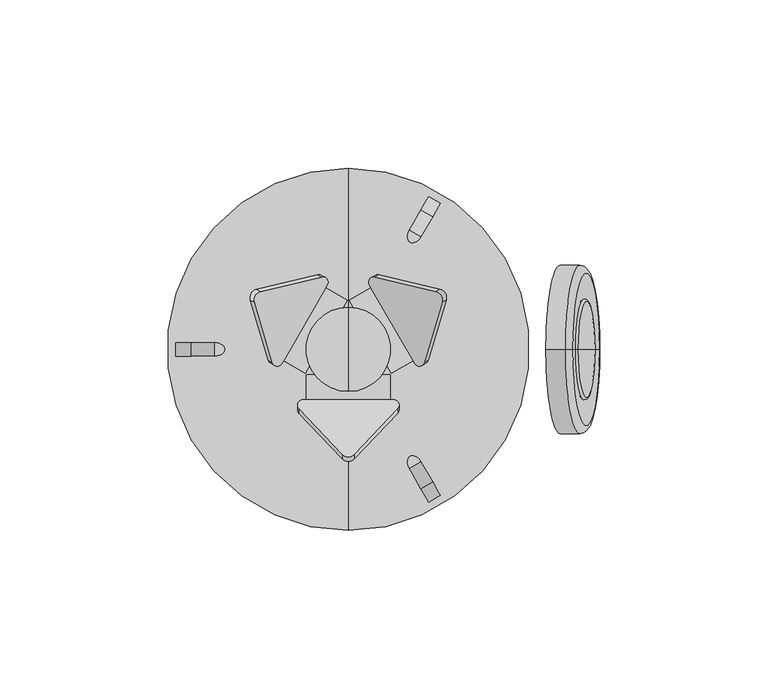
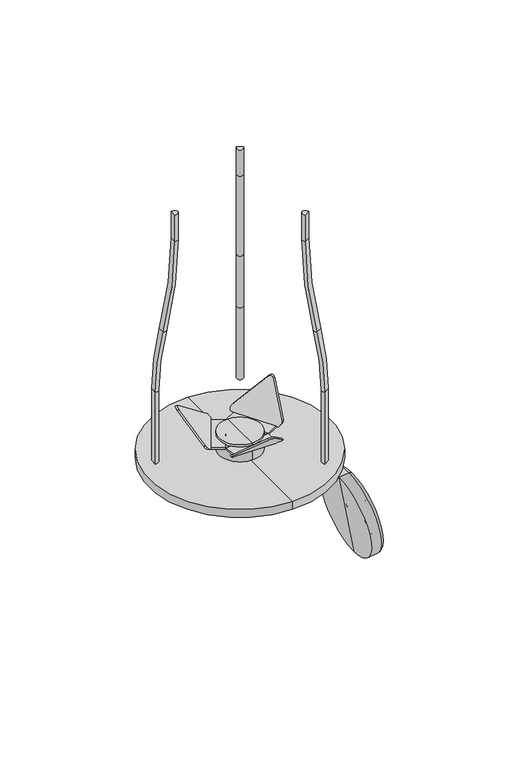
"""IFC4 building model written with IfcOpenShell, lengths in millimetres: proxy geometry, Smoothie_Maker_ : Smoothie_Maker_."""

from ifc_helpers import new_model, si_unit, point, frame, origin, place, context, project, spatial, polyline, circle_curve, ellipse_curve, trimmed, source, transform, mapped, element, save
from ifc_brep_helpers import plane_surface, cylinder_surface, revolved_surface, extruded_surface, advanced_brep


def generic_models_17cbc278(model_context):
    return source(origin(), model_context, "Body", "AdvancedBrep", [
        advanced_brep(
        [(21.5767384, -33.401336, 302.0), (18.1380363, -35.3866715, 302.0), (21.5767384, -33.401336, 285.575084), (18.1380363, -35.3866715, 285.575084), (21.6115055, -41.4028966, 231.2107577), (25.0502075, -39.417561, 231.2107577), (23.9250989, -45.410158, 195.0), (27.363801, -43.4248225, 195.0), (27.363801, -43.4248225, 150.0), (23.9250989, -45.410158, 150.0)],
        [
            (0, 1, ellipse_curve(frame((19.8573873, -34.3940038, 302.0), z_axis=(0.0, 0.0, 1.0), x_axis=(0.5000000000000502, -0.8660254037844097, 0.0)), 2.9839648, 1.9853355)),
            (1, 0),
            (0, 2),
            (2, 3, ellipse_curve(frame((19.8573873, -34.3940038, 285.575084), z_axis=(0.0, 0.0, 1.0), x_axis=(0.5000000000000502, -0.8660254037844097, 0.0)), 2.9839648, 1.9853355)),
            (3, 1),
            (3, 2),
            (4, 3, circle_curve(frame((126.233855, -222.6141215, 285.575084), z_axis=(0.8660254037844424, 0.49999999999999367, 0.0), x_axis=(-0.49999999999999367, 0.8660254037844424, 0.0)), 216.1916373)),
            (2, 5, circle_curve(frame((129.672557, -220.628786, 285.575084), z_axis=(-0.8660254037844424, -0.49999999999999367, 0.0), x_axis=(-0.49999999999999367, 0.8660254037844424, 0.0)), 216.1916373)),
            (5, 4, ellipse_curve(frame((23.3308565, -40.4102288, 231.2107577), z_axis=(-0.1257317975289871, 0.2177738614471723, 0.9678667575449205), x_axis=(0.4839333787725105, -0.838197199512346, 0.25146359505797733)), 2.9839648, 1.9853355)),
            (4, 5),
            (6, 4, circle_curve(frame((-48.0749011, 79.2975001, 195.0), z_axis=(-0.8660254037844424, -0.49999999999999367, 0.0), x_axis=(0.4839333787724538, -0.8381971995123781, 0.25146359505797933)), 144.0)),
            (5, 7, circle_curve(frame((-44.636199, 81.2828357, 195.0), z_axis=(0.8660254037844424, 0.49999999999999367, 0.0), x_axis=(0.4839333787724538, -0.8381971995123781, 0.25146359505797933)), 144.0)),
            (7, 6, ellipse_curve(frame((25.6444499, -44.4174902, 195.0), z_axis=(0.0, 0.0, 1.0), x_axis=(0.5000000000000503, -0.8660254037844097, 0.0)), 2.9839648, 1.9853355)),
            (6, 7),
            (8, 9),
            (9, 8, ellipse_curve(frame((25.6444499, -44.4174902, 150.0), z_axis=(0.0, 0.0, -1.0), x_axis=(0.5000000000000503, -0.8660254037844097, 0.0)), 2.9839648, 1.9853355)),
            (7, 8),
            (9, 6),
        ],
        [
            plane_surface(frame((19.8573873, -34.3940038, 302.0), z_axis=(0.0, 0.0, 1.0), x_axis=(0.8660254037844424, 0.4999999999999936, 0.0))),
            extruded_surface(trimmed(ellipse_curve(frame((19.8573873, -34.3940038, 285.575084), z_axis=(0.0, 0.0, 1.0), x_axis=(0.5000000000000502, -0.8660254037844097, 0.0)), 2.9839648, 1.9853355), [point((21.5767384, -33.401336, 285.575084))], [point((18.1380363, -35.3866715, 285.575084))], True, "CARTESIAN"), (0.0, 0.0, 16.424915999999996), 16.424915999999996),
            plane_surface(frame((18.1380363, -35.3866715, 302.0), z_axis=(0.49999999999999545, -0.8660254037844413, 0.0), x_axis=(0.0, 0.0, -1.0))),
            revolved_surface(trimmed(ellipse_curve(frame((19.8573873, -34.3940038, 285.575084), z_axis=(0.0, 0.0, 1.0), x_axis=(0.5000000000000502, -0.8660254037844097, 0.0)), 2.9839648, 1.9853355), [point((21.5767384, -33.401336, 285.575084))], [point((18.1380363, -35.3866715, 285.575084))], True, "CARTESIAN"), (127.953206, -221.6214537, 285.575084), (-0.8660254037844424, -0.49999999999999367, 0.0)),
            revolved_surface(polyline([(18.13803630173097, -35.38667150299814, 285.575084), (21.576738365748525, -33.40133594067472, 285.575084)]), (127.953206, -221.6214537, 285.575084), (-0.8660254037844424, -0.49999999999999367, 0.0)),
            revolved_surface(trimmed(ellipse_curve(frame((23.3308565, -40.4102288, 231.2107577), z_axis=(-0.12573179752898733, 0.21777386144717267, 0.9678667575449205), x_axis=(0.48393337877251064, -0.8381971995123458, 0.2514635950579777)), 2.9839648, 1.9853355), [point((25.0502075, -39.417561, 231.2107577))], [point((21.6115055, -41.4028966, 231.2107577))], True, "CARTESIAN"), (-46.3555501, 80.2901679, 195.0), (0.8660254037844424, 0.49999999999999367, 0.0)),
            cylinder_surface(frame((-46.3555501, 80.2901679, 195.0), z_axis=(0.8660254037844424, 0.49999999999999367, 0.0), x_axis=(0.4839333787724538, -0.8381971995123781, 0.25146359505797933)), 144.0),
            plane_surface(frame((25.6444499, -44.4174902, 150.0), z_axis=(0.0, 0.0, -1.0), x_axis=(0.8660254037844424, 0.49999999999999367, 0.0))),
            extruded_surface(trimmed(ellipse_curve(frame((25.6444499, -44.4174902, 150.0), z_axis=(0.0, 0.0, 1.0), x_axis=(0.5000000000000503, -0.8660254037844097, 0.0)), 2.9839648, 1.9853355), [point((27.363801, -43.4248225, 150.0))], [point((23.9250989, -45.410158, 150.0))], True, "CARTESIAN"), (0.0, 0.0, 45.0), 45.0),
            plane_surface(frame((23.9250989, -45.410158, 195.0), z_axis=(0.49999999999999545, -0.8660254037844413, 0.0), x_axis=(0.0, 0.0, -1.0))),
        ],
        [
            (0, [[1, 2]]),
            (1, [[-1, 3, 4, 5]]),
            (2, [[-2, -5, 6, -3]]),
            (3, [[7, -4, 8, 9]]),
            (4, [[-8, -6, -7, 10]]),
            (5, [[11, -9, 12, 13]]),
            (6, [[-12, -10, -11, 14]]),
            (7, [[15, 16]]),
            (8, [[-13, 17, -16, 18]]),
            (9, [[-14, -18, -15, -17]]),
        ],
    ),
        advanced_brep(
        [(18.1380363, 35.3866715, 302.0), (21.5767384, 33.401336, 302.0), (18.1380363, 35.3866715, 285.575084), (21.5767384, 33.401336, 285.575084), (25.0502075, 39.417561, 231.2107577), (21.6115055, 41.4028966, 231.2107577), (27.363801, 43.4248225, 195.0), (23.9250989, 45.410158, 195.0), (23.9250989, 45.410158, 150.0), (27.363801, 43.4248225, 150.0)],
        [
            (0, 1, ellipse_curve(frame((19.8573873, 34.3940038, 302.0), z_axis=(0.0, 0.0, 1.0), x_axis=(0.4999999999999584, 0.8660254037844627, 0.0)), 2.9839648, 1.9853355)),
            (1, 0),
            (0, 2),
            (2, 3, ellipse_curve(frame((19.8573873, 34.3940038, 285.575084), z_axis=(0.0, 0.0, 1.0), x_axis=(0.4999999999999584, 0.8660254037844627, 0.0)), 2.9839648, 1.9853355)),
            (3, 1),
            (3, 2),
            (4, 3, circle_curve(frame((129.672557, 220.628786, 285.575084), z_axis=(-0.86602540378443, 0.500000000000015, 0.0), x_axis=(-0.500000000000015, -0.86602540378443, 0.0)), 216.1916373)),
            (2, 5, circle_curve(frame((126.233855, 222.6141215, 285.575084), z_axis=(0.86602540378443, -0.500000000000015, 0.0), x_axis=(-0.500000000000015, -0.86602540378443, 0.0)), 216.1916373)),
            (5, 4, ellipse_curve(frame((23.3308565, 40.4102288, 231.2107577), z_axis=(-0.12573179752899238, -0.2177738614471692, 0.9678667575449205), x_axis=(0.4839333787724181, 0.8381971995123993, 0.2514635950579773)), 2.9839648, 1.9853355)),
            (4, 5),
            (6, 4, circle_curve(frame((-44.636199, -81.2828357, 195.0), z_axis=(0.86602540378443, -0.500000000000015, 0.0), x_axis=(0.4839333787724744, 0.8381971995123663, 0.25146359505797933)), 144.0)),
            (5, 7, circle_curve(frame((-48.0749011, -79.2975001, 195.0), z_axis=(-0.86602540378443, 0.500000000000015, 0.0), x_axis=(0.4839333787724744, 0.8381971995123663, 0.25146359505797933)), 144.0)),
            (7, 6, ellipse_curve(frame((25.6444499, 44.4174902, 195.0), z_axis=(0.0, 0.0, 1.0), x_axis=(0.4999999999999585, 0.8660254037844627, 0.0)), 2.9839648, 1.9853355)),
            (6, 7),
            (8, 9),
            (9, 8, ellipse_curve(frame((25.6444499, 44.4174902, 150.0), z_axis=(0.0, 0.0, -0.9999999999999998), x_axis=(0.49999999999995837, 0.8660254037844626, 0.0)), 2.9839648, 1.9853355)),
            (7, 8),
            (9, 6),
        ],
        [
            plane_surface(frame((19.8573873, 34.3940038, 302.0), z_axis=(0.0, 0.0, 1.0), x_axis=(-0.86602540378443, 0.500000000000015, 0.0))),
            extruded_surface(trimmed(ellipse_curve(frame((19.8573873, 34.3940038, 285.575084), z_axis=(0.0, 0.0, 1.0), x_axis=(0.4999999999999584, 0.8660254037844627, 0.0)), 2.9839648, 1.9853355), [point((18.1380363, 35.3866715, 285.575084))], [point((21.5767384, 33.401336, 285.575084))], True, "CARTESIAN"), (0.0, 0.0, 16.424915999999996), 16.424915999999996),
            plane_surface(frame((21.5767384, 33.401336, 302.0), z_axis=(0.5000000000000131, 0.8660254037844312, 0.0), x_axis=(0.0, 0.0, -1.0))),
            revolved_surface(trimmed(ellipse_curve(frame((19.8573873, 34.3940038, 285.575084), z_axis=(0.0, 0.0, 1.0), x_axis=(0.4999999999999584, 0.8660254037844627, 0.0)), 2.9839648, 1.9853355), [point((18.1380363, 35.3866715, 285.575084))], [point((21.5767384, 33.401336, 285.575084))], True, "CARTESIAN"), (127.953206, 221.6214537, 285.575084), (0.86602540378443, -0.500000000000015, 0.0)),
            revolved_surface(polyline([(21.57673836574851, 33.401335940674684, 285.575084), (18.138036301730992, 35.3866715029982, 285.575084)]), (127.953206, 221.6214537, 285.575084), (0.86602540378443, -0.500000000000015, 0.0)),
            revolved_surface(trimmed(ellipse_curve(frame((23.3308565, 40.4102288, 231.2107577), z_axis=(-0.1257317975289926, -0.2177738614471695, 0.9678667575449204), x_axis=(0.4839333787724181, 0.8381971995123992, 0.25146359505797766)), 2.9839648, 1.9853355), [point((21.6115055, 41.4028966, 231.2107577))], [point((25.0502075, 39.417561, 231.2107577))], True, "CARTESIAN"), (-46.3555501, -80.2901679, 195.0), (-0.86602540378443, 0.500000000000015, 0.0)),
            cylinder_surface(frame((-46.3555501, -80.2901679, 195.0), z_axis=(-0.86602540378443, 0.500000000000015, 0.0), x_axis=(0.4839333787724744, 0.8381971995123663, 0.25146359505797933)), 144.0),
            plane_surface(frame((25.6444499, 44.4174902, 150.0), z_axis=(0.0, 0.0, -1.0), x_axis=(-0.86602540378443, 0.500000000000015, 0.0))),
            extruded_surface(trimmed(ellipse_curve(frame((25.6444499, 44.4174902, 150.0), z_axis=(0.0, 0.0, 0.9999999999999998), x_axis=(0.49999999999995837, 0.8660254037844626, 0.0)), 2.9839648, 1.9853355), [point((23.9250989, 45.410158, 150.0))], [point((27.363801, 43.4248225, 150.0))], True, "CARTESIAN"), (0.0, 0.0, 45.0), 45.0),
            plane_surface(frame((27.363801, 43.4248225, 195.0), z_axis=(0.5000000000000132, 0.8660254037844312, 0.0), x_axis=(0.0, 0.0, -1.0))),
        ],
        [
            (0, [[1, 2]]),
            (1, [[-1, 3, 4, 5]]),
            (2, [[-2, -5, 6, -3]]),
            (3, [[7, -4, 8, 9]]),
            (4, [[-8, -6, -7, 10]]),
            (5, [[11, -9, 12, 13]]),
            (6, [[-12, -10, -11, 14]]),
            (7, [[15, 16]]),
            (8, [[-13, 17, -16, 18]]),
            (9, [[-14, -18, -15, -17]]),
        ],
    ),
        advanced_brep(
        [(-39.7147747, -1.9853355, 302.0), (-39.7147747, 1.9853355, 302.0), (-39.7147747, -1.9853355, 285.575084), (-39.7147747, 1.9853355, 285.575084), (-46.661713, 1.9853355, 231.2107577), (-46.661713, -1.9853355, 231.2107577), (-51.2888999, 1.9853355, 195.0), (-51.2888999, -1.9853355, 195.0), (-51.2888999, -1.9853355, 150.0), (-51.2888999, 1.9853355, 150.0)],
        [
            (0, 1, ellipse_curve(frame((-39.7147747, 0.0, 302.0), z_axis=(0.0, 0.0, 1.0), x_axis=(-1.0, 0.0, 0.0)), 2.9839648, 1.9853355)),
            (1, 0),
            (0, 2),
            (2, 3, ellipse_curve(frame((-39.7147747, 0.0, 285.575084), z_axis=(0.0, 0.0, 1.0), x_axis=(-1.0, 0.0, 0.0)), 2.9839648, 1.9853355)),
            (3, 1),
            (3, 2),
            (4, 3, circle_curve(frame((-255.9064119, 1.9853355, 285.575084), z_axis=(0.0, -1.0, 0.0), x_axis=(1.0, 0.0, 0.0)), 216.1916373)),
            (2, 5, circle_curve(frame((-255.9064119, -1.9853355, 285.575084), z_axis=(0.0, 1.0, 0.0), x_axis=(1.0, 0.0, 0.0)), 216.1916373)),
            (5, 4, ellipse_curve(frame((-46.661713, 0.0, 231.2107577), z_axis=(0.25146359505797744, 0.0, 0.9678667575449205), x_axis=(-0.9678667575449202, 0.0, 0.2514635950579774)), 2.9839648, 1.9853355)),
            (4, 5),
            (6, 4, circle_curve(frame((92.7111001, 1.9853355, 195.0), z_axis=(0.0, 1.0, 0.0), x_axis=(-0.9678667575449198, 0.0, 0.25146359505797933)), 144.0)),
            (5, 7, circle_curve(frame((92.7111001, -1.9853355, 195.0), z_axis=(0.0, -1.0, 0.0), x_axis=(-0.9678667575449198, 0.0, 0.25146359505797933)), 144.0)),
            (7, 6, ellipse_curve(frame((-51.2888999, 0.0, 195.0), z_axis=(0.0, 0.0, 1.0), x_axis=(-0.9999999999999999, 0.0, 0.0)), 2.9839648, 1.9853355)),
            (6, 7),
            (8, 9),
            (9, 8, ellipse_curve(frame((-51.2888999, 0.0, 150.0), z_axis=(0.0, 0.0, -1.0), x_axis=(-1.0, 0.0, 0.0)), 2.9839648, 1.9853355)),
            (7, 8),
            (9, 6),
        ],
        [
            plane_surface(frame((-39.7147747, 0.0, 302.0), z_axis=(0.0, 0.0, 1.0), x_axis=(0.0, -1.0, 0.0))),
            extruded_surface(trimmed(ellipse_curve(frame((-39.7147747, 0.0, 285.575084), z_axis=(0.0, 0.0, 1.0), x_axis=(-1.0, 0.0, 0.0)), 2.9839648, 1.9853355), [point((-39.7147747, -1.9853355, 285.575084))], [point((-39.7147747, 1.9853355, 285.575084))], True, "CARTESIAN"), (0.0, 0.0, 16.424915999999996), 16.424915999999996),
            plane_surface(frame((-39.7147747, 1.9853355, 302.0), z_axis=(-1.0, 0.0, 0.0), x_axis=(0.0, 0.0, -1.0))),
            revolved_surface(trimmed(ellipse_curve(frame((-39.7147747, 0.0, 285.575084), z_axis=(0.0, 0.0, 1.0), x_axis=(-1.0, 0.0, 0.0)), 2.9839648, 1.9853355), [point((-39.7147747, -1.9853355, 285.575084))], [point((-39.7147747, 1.9853355, 285.575084))], True, "CARTESIAN"), (-255.9064119, 0.0, 285.575084), (0.0, 1.0, 0.0)),
            revolved_surface(polyline([(-39.7147746, 1.9853355, 285.575084), (-39.7147746, -1.9853355, 285.575084)]), (-255.9064119, 0.0, 285.575084), (0.0, 1.0, 0.0)),
            revolved_surface(trimmed(ellipse_curve(frame((-46.661713, 0.0, 231.2107577), z_axis=(0.25146359505797766, 0.0, 0.9678667575449202), x_axis=(-0.9678667575449202, 0.0, 0.25146359505797766)), 2.9839648, 1.9853355), [point((-46.661713, -1.9853355, 231.2107577))], [point((-46.661713, 1.9853355, 231.2107577))], True, "CARTESIAN"), (92.7111001, 0.0, 195.0), (0.0, -1.0, 0.0)),
            cylinder_surface(frame((92.7111001, 0.0, 195.0), z_axis=(0.0, -1.0, 0.0), x_axis=(-0.9678667575449198, 0.0, 0.25146359505797933)), 144.0),
            plane_surface(frame((-51.2888999, 0.0, 150.0), z_axis=(0.0, 0.0, -1.0), x_axis=(0.0, -1.0, 0.0))),
            extruded_surface(trimmed(ellipse_curve(frame((-51.2888999, 0.0, 150.0), z_axis=(0.0, 0.0, 1.0), x_axis=(-1.0, 0.0, 0.0)), 2.9839648, 1.9853355), [point((-51.2888999, -1.9853355, 150.0))], [point((-51.2888999, 1.9853355, 150.0))], True, "CARTESIAN"), (0.0, 0.0, 45.0), 45.0),
            plane_surface(frame((-51.2888999, 1.9853355, 195.0), z_axis=(-1.0, 0.0, 0.0), x_axis=(0.0, 0.0, -1.0))),
        ],
        [
            (0, [[1, 2]]),
            (1, [[-1, 3, 4, 5]]),
            (2, [[-2, -5, 6, -3]]),
            (3, [[7, -4, 8, 9]]),
            (4, [[-8, -6, -7, 10]]),
            (5, [[11, -9, 12, 13]]),
            (6, [[-12, -10, -11, 14]]),
            (7, [[15, 16]]),
            (8, [[-13, 17, -16, 18]]),
            (9, [[-14, -18, -15, -17]]),
        ],
    ),
        advanced_brep(
        [(73.3589669, 0.0, 64.6121124), (68.4033068, 0.0, 92.7170578), (70.8811368, 0.0, 78.6645851), (71.9196798, 0.0, 64.3583272), (66.9640196, 0.0, 92.4632727), (69.4418497, 0.0, 78.4108)],
        [
            (0, 1, circle_curve(frame((70.8811368, 0.0, 78.6645851), z_axis=(0.9848077530122592, 0.0, 0.1736481776666406), x_axis=(-0.1736481776666406, 0.0, 0.9848077530122592)), 14.2692548)),
            (1, 2),
            (2, 0),
            (1, 0, circle_curve(frame((70.8811368, 0.0, 78.6645851), z_axis=(0.9848077530122592, 0.0, 0.1736481776666406), x_axis=(-0.1736481776666406, 0.0, 0.9848077530122592)), 14.2692548)),
            (3, 4, circle_curve(frame((69.4418497, 0.0, 78.4108), z_axis=(0.9848077530122592, 0.0, 0.1736481776666406), x_axis=(-0.1736481776666406, 0.0, 0.9848077530122592)), 14.2692548)),
            (4, 1, circle_curve(frame((67.6836632, 0.0, 92.5901653), z_axis=(0.0, 1.0, 0.0), x_axis=(1.0, 0.0, 0.0)), 0.7307452)),
            (0, 3, circle_curve(frame((72.6393234, 0.0, 64.4852198), z_axis=(0.0, 1.0, 0.0), x_axis=(0.9396926207861097, 0.0, 0.34202014332511577)), 0.7307452)),
            (4, 3, circle_curve(frame((69.4418497, 0.0, 78.4108), z_axis=(0.9848077530122592, 0.0, 0.1736481776666406), x_axis=(-0.1736481776666406, 0.0, 0.9848077530122592)), 14.2692548)),
            (5, 4),
            (3, 5),
        ],
        [
            plane_surface(frame((70.8811368, 0.0, 78.6645851), z_axis=(0.9848077530122592, 0.0, 0.1736481776666406), x_axis=(-0.1736481776666406, 0.0, 0.9848077530122592))),
            revolved_surface(trimmed(ellipse_curve(frame((67.6836632, 0.0, 92.5901653), z_axis=(0.0, -1.0, 0.0), x_axis=(1.0, 0.0, 0.0)), 0.7307452, 0.7307452), [point((68.4033068, 0.0, 92.7170578))], [point((66.9640196, 0.0, 92.4632727))], True, "CARTESIAN"), (69.4418497, 0.0, 78.4108), (-0.9848077530122592, 0.0, -0.1736481776666406)),
            plane_surface(frame((69.4418497, 0.0, 78.4108), z_axis=(-0.9848077530122592, 0.0, -0.1736481776666406), x_axis=(-0.1736481776666406, 0.0, 0.9848077530122592))),
        ],
        [
            (0, [[1, 2, 3]]),
            (0, [[4, -3, -2]]),
            (1, [[5, 6, -1, 7]]),
            (1, [[8, -7, -4, -6]]),
            (2, [[9, -5, 10]]),
            (2, [[-10, -8, -9]]),
        ],
    ),
        advanced_brep(
        [(63.0405993, 0.0, 77.2820868), (58.6994009, 0.0, 101.9022467), (67.3817978, 0.0, 52.6619269), (64.4343413, 0.0, 102.9134714), (73.1167382, 0.0, 53.6731517), (74.6597308, 0.0, 56.2960724), (66.7813718, 0.0, 100.9764668), (68.9494458, 0.0, 78.3239759)],
        [
            (0, 1),
            (1, 2, circle_curve(frame((63.0405993, 0.0, 77.2820868), z_axis=(-0.9848077530122603, 0.0, -0.1736481776666345), x_axis=(-0.1736481776666345, 0.0, 0.9848077530122603)), 24.9999655)),
            (2, 0),
            (2, 1, circle_curve(frame((63.0405993, 0.0, 77.2820868), z_axis=(-0.9848077530122603, 0.0, -0.1736481776666345), x_axis=(-0.1736481776666345, 0.0, 0.9848077530122603)), 24.9999655)),
            (1, 3),
            (3, 4, circle_curve(frame((68.7755398, 0.0, 78.2933115), z_axis=(-0.9848077530122603, 0.0, -0.1736481776666345), x_axis=(-0.1736481776666345, 0.0, 0.9848077530122603)), 24.9999655)),
            (4, 2),
            (4, 3, circle_curve(frame((68.7755398, 0.0, 78.2933115), z_axis=(-0.9848077530122603, 0.0, -0.1736481776666345), x_axis=(-0.1736481776666345, 0.0, 0.9848077530122603)), 24.9999655)),
            (5, 6, circle_curve(frame((70.7205513, 0.0, 78.6362696), z_axis=(0.9848077530122603, 0.0, 0.1736481776666345), x_axis=(-0.1736481776666345, 0.0, 0.9848077530122603)), 22.6848307)),
            (6, 7, circle_curve(frame((210.7312959, 0.0, 103.3239414), z_axis=(0.0, -1.0000000000000002, 0.0), x_axis=(1.0000000000000002, 0.0, 0.0)), 143.9690637)),
            (7, 5, circle_curve(frame((210.7312959, 0.0, 103.3239414), z_axis=(0.0, -1.0000000000000002, 0.0), x_axis=(0.939692620786114, 0.0, 0.3420201433251042)), 143.9690637)),
            (6, 5, circle_curve(frame((70.7205513, 0.0, 78.6362696), z_axis=(0.9848077530122603, 0.0, 0.1736481776666345), x_axis=(-0.1736481776666345, 0.0, 0.9848077530122603)), 22.6848307)),
            (3, 6, circle_curve(frame((64.7816377, 0.0, 100.9438559), z_axis=(0.0, 1.0000000000000002, 0.0), x_axis=(1.0000000000000002, 0.0, 0.0)), 2.0)),
            (5, 4, circle_curve(frame((72.7694419, 0.0, 55.6427672), z_axis=(0.0, 1.0000000000000002, 0.0), x_axis=(0.939692620786114, 0.0, 0.3420201433251042)), 2.0)),
        ],
        [
            plane_surface(frame((63.0405993, 0.0, 77.2820868), z_axis=(-0.9848077530122603, 0.0, -0.1736481776666345), x_axis=(-0.1736481776666345, 0.0, 0.9848077530122603))),
            cylinder_surface(frame((68.9494458, 0.0, 78.3239759), z_axis=(-0.9848077530122603, 0.0, -0.1736481776666345), x_axis=(-0.1736481776666345, 0.0, 0.9848077530122603)), 24.9999655),
            revolved_surface(trimmed(ellipse_curve(frame((210.7312959, 0.0, 103.3239414), z_axis=(0.0, 1.0000000000000002, 0.0), x_axis=(1.0000000000000002, 0.0, 0.0)), 143.9690637, 143.9690637), [point((68.9494458, 0.0, 78.3239759))], [point((66.7813718, 0.0, 100.9764668))], True, "CARTESIAN"), (68.9494458, 0.0, 78.3239759), (-0.9848077530122603, 0.0, -0.1736481776666345)),
            revolved_surface(trimmed(ellipse_curve(frame((64.7816377, 0.0, 100.9438559), z_axis=(0.0, -1.0000000000000002, 0.0), x_axis=(1.0000000000000002, 0.0, 0.0)), 2.0, 2.0), [point((66.7813718, 0.0, 100.9764668))], [point((64.4343413, 0.0, 102.9134714))], True, "CARTESIAN"), (68.9494458, 0.0, 78.3239759), (-0.9848077530122603, 0.0, -0.1736481776666345)),
        ],
        [
            (0, [[1, 2, 3]]),
            (0, [[-3, 4, -1]]),
            (1, [[-2, 5, 6, 7]]),
            (1, [[-4, -7, 8, -5]]),
            (2, [[9, 10, 11]]),
            (2, [[12, -11, -10]]),
            (3, [[-6, 13, -9, 14]]),
            (3, [[-8, -14, -12, -13]]),
        ],
    ),
        advanced_brep(
        [(6.7403811, 18.3253175, 150.0), (19.2403811, -3.3253175, 150.0), (19.763146, -4.230773, 150.0), (22.5545844, -3.961988, 152.5518491), (27.8680358, 13.9604825, 166.1146682), (26.0241504, 17.1541857, 166.1146682), (7.8461099, 21.5138371, 152.5518491), (6.2176161, 19.230773, 150.0), (19.5991005, -3.1182108, 149.0), (7.0991005, 18.5324243, 149.0), (7.9651259, 19.0324243, 150.0), (7.442361, 19.9378797, 150.0), (9.0708548, 22.2209439, 152.5518491), (27.2488952, 17.8612925, 166.1146682), (29.0927807, 14.6675893, 166.1146682), (23.7793293, -3.2548812, 152.5518491), (20.9878909, -3.5236662, 150.0), (20.4651259, -2.6182108, 150.0), (12.7451905, -7.0753175, 149.0), (0.2451905, 14.5753175, 149.0), (12.7451905, -7.0753175, 150.0), (0.2451905, 14.5753175, 150.0)],
        [
            (0, 1),
            (1, 2),
            (2, 3, ellipse_curve(frame((21.097619, -3.4603146, 151.5409167), z_axis=(-0.6123724356957986, -0.35355339059327007, 0.7071067811865459), x_axis=(-0.6123724356957957, -0.35355339059326846, -0.7071067811865492)), 2.1791853, 1.5409167)),
            (3, 4),
            (4, 5, ellipse_curve(frame((25.4314493, 14.6828541, 164.3657082), z_axis=(-0.6123724356957986, -0.35355339059327007, 0.7071067811865459), x_axis=(-0.6123724356957957, -0.35355339059326846, -0.7071067811865492)), 3.5940992, 2.5414119)),
            (5, 6),
            (6, 7, ellipse_curve(frame((7.5520892, 20.0012313, 151.5409167), z_axis=(-0.6123724356957986, -0.35355339059327007, 0.7071067811865459), x_axis=(-0.6123724356957957, -0.35355339059326846, -0.7071067811865492)), 2.1791853, 1.5409167)),
            (7, 0),
            (8, 9),
            (9, 10),
            (10, 11),
            (11, 12, ellipse_curve(frame((8.776834, 20.7083381, 151.5409167), z_axis=(0.6123724356957986, 0.35355339059327007, -0.7071067811865459), x_axis=(-0.6123724356957957, -0.35355339059326846, -0.7071067811865492)), 2.1791853, 1.5409167)),
            (12, 13),
            (13, 14, ellipse_curve(frame((26.6561941, 15.3899609, 164.3657082), z_axis=(0.6123724356957986, 0.35355339059327007, -0.7071067811865459), x_axis=(-0.6123724356957957, -0.35355339059326846, -0.7071067811865492)), 3.5940992, 2.5414119)),
            (14, 15),
            (15, 16, ellipse_curve(frame((22.3223639, -2.7532078, 151.5409167), z_axis=(0.6123724356957986, 0.35355339059327007, -0.7071067811865459), x_axis=(-0.6123724356957957, -0.35355339059326846, -0.7071067811865492)), 2.1791853, 1.5409167)),
            (16, 17),
            (17, 8),
            (8, 18),
            (18, 19),
            (19, 9),
            (18, 20),
            (20, 21),
            (21, 19),
            (0, 21),
            (20, 1),
            (7, 11),
            (10, 0),
            (17, 1),
            (16, 2),
            (15, 3),
            (14, 4),
            (13, 5),
            (12, 6),
        ],
        [
            plane_surface(frame((2.9903811, 24.8205081, 150.0), z_axis=(-0.6123724356957987, -0.3535533905932701, 0.707106781186546), x_axis=(0.49999999999999367, -0.8660254037844424, 0.0))),
            plane_surface(frame((18.9120644, 34.0128962, 166.9705627), z_axis=(0.6123724356957987, 0.3535533905932701, -0.707106781186546), x_axis=(0.49999999999999367, -0.8660254037844424, 0.0))),
            plane_surface(frame((3.3491005, 25.0276149, 149.0), z_axis=(1.745941772753253e-12, 1.0080199524884858e-12, -1.0), x_axis=(0.49999999999999356, -0.8660254037844424, 0.0))),
            plane_surface(frame((-3.5048095, 21.0705081, 149.0), z_axis=(-0.8660254037844424, -0.49999999999999367, 0.0), x_axis=(0.49999999999999367, -0.8660254037844424, 0.0))),
            plane_surface(frame((-3.5048095, 21.0705081, 150.0), z_axis=(-1.7466346998929444e-12, -1.0084200141591156e-12, 1.0), x_axis=(0.49999999999999367, -0.8660254037844424, 0.0))),
            plane_surface(frame((24.3155526, 29.6796215, 150.0), z_axis=(-2.5488208859774175e-12, 4.414687273905682e-12, -1.0000000000000002), x_axis=(-0.8660254037844424, -0.4999999999999937, 0.0))),
            plane_surface(frame((24.8383175, 28.774166, 150.0), z_axis=(-0.4999999999999936, 0.8660254037844424, 0.0), x_axis=(-0.8660254037844424, -0.4999999999999936, 0.0))),
            plane_surface(frame((37.3383175, 7.1235309, 149.0), z_axis=(0.4999999999999936, -0.8660254037844424, 0.0), x_axis=(-0.8660254037844424, -0.4999999999999936, 0.0))),
            plane_surface(frame((37.3383175, 7.1235309, 150.0), z_axis=(2.556912380853556e-12, -4.428702154140338e-12, -1.0), x_axis=(-0.8660254037844424, -0.49999999999999367, 0.0))),
            cylinder_surface(frame((13.2679555, -7.980773, 151.5409167), z_axis=(-0.8660254037844424, -0.49999999999999367, 0.0), x_axis=(-0.49999999999999367, 0.8660254037844424, 0.0)), 1.5409167),
            plane_surface(frame((38.4425548, 5.2109359, 152.5518491), z_axis=(0.36276791776973083, -0.6283324649331531, 0.6881843876084679), x_axis=(-0.8660254037844424, -0.4999999999999936, 0.0))),
            cylinder_surface(frame((6.4951905, 3.75, 164.3657082), z_axis=(-0.8660254037844424, -0.49999999999999367, 0.0), x_axis=(-0.49999999999999367, 0.8660254037844424, 0.0)), 2.5414119),
            plane_surface(frame((30.1663748, 19.5457001, 166.1146682), z_axis=(-0.3627679177697329, 0.6283324649331566, 0.6881843876084636), x_axis=(-0.8660254037844424, -0.4999999999999936, 0.0))),
            cylinder_surface(frame((-0.2775744, 15.480773, 151.5409167), z_axis=(-0.8660254037844424, -0.49999999999999367, 0.0), x_axis=(0.49999999999999367, -0.8660254037844424, 0.0)), 1.5409167),
        ],
        [
            (0, [[1, 2, 3, 4, 5, 6, 7, 8]]),
            (1, [[9, 10, 11, 12, 13, 14, 15, 16, 17, 18]]),
            (2, [[-9, 19, 20, 21]]),
            (3, [[-20, 22, 23, 24]]),
            (4, [[-1, 25, -23, 26]]),
            (5, [[27, -11, 28, -8]]),
            (6, [[-28, -10, -21, -24, -25]]),
            (7, [[29, -26, -22, -19, -18]]),
            (8, [[-29, -17, 30, -2]]),
            (9, [[-30, -16, 31, -3]]),
            (10, [[-31, -15, 32, -4]]),
            (11, [[-32, -14, 33, -5]]),
            (12, [[-33, -13, 34, -6]]),
            (13, [[-27, -7, -34, -12]]),
        ],
    ),
        advanced_brep(
        [(-19.2403811, -3.3253175, 150.0), (-6.7403811, 18.3253175, 150.0), (-6.2176161, 19.230773, 150.0), (-7.8461099, 21.5138371, 152.5518491), (-26.0241504, 17.1541857, 166.1146682), (-27.8680358, 13.9604825, 166.1146682), (-22.5545844, -3.961988, 152.5518491), (-19.763146, -4.230773, 150.0), (-7.0991005, 18.5324243, 149.0), (-19.5991005, -3.1182108, 149.0), (-20.4651259, -2.6182108, 150.0), (-20.9878909, -3.5236662, 150.0), (-23.7793293, -3.2548812, 152.5518491), (-29.0927807, 14.6675893, 166.1146682), (-27.2488952, 17.8612925, 166.1146682), (-9.0708548, 22.2209439, 152.5518491), (-7.442361, 19.9378797, 150.0), (-7.9651259, 19.0324243, 150.0), (-0.2451905, 14.5753175, 149.0), (-12.7451905, -7.0753175, 149.0), (-0.2451905, 14.5753175, 150.0), (-12.7451905, -7.0753175, 150.0)],
        [
            (0, 1),
            (1, 2),
            (2, 3, ellipse_curve(frame((-7.5520892, 20.0012313, 151.5409167), z_axis=(0.6123724356957898, -0.35355339059328517, 0.7071067811865459), x_axis=(0.612372435695787, -0.3535533905932836, -0.7071067811865491)), 2.1791853, 1.5409167)),
            (3, 4),
            (4, 5, ellipse_curve(frame((-25.4314493, 14.6828541, 164.3657082), z_axis=(0.6123724356957898, -0.35355339059328517, 0.7071067811865459), x_axis=(0.612372435695787, -0.3535533905932836, -0.7071067811865491)), 3.5940992, 2.5414119)),
            (5, 6),
            (6, 7, ellipse_curve(frame((-21.097619, -3.4603146, 151.5409167), z_axis=(0.6123724356957898, -0.35355339059328517, 0.7071067811865459), x_axis=(0.612372435695787, -0.3535533905932836, -0.7071067811865491)), 2.1791853, 1.5409167)),
            (7, 0),
            (8, 9),
            (9, 10),
            (10, 11),
            (11, 12, ellipse_curve(frame((-22.3223639, -2.7532078, 151.5409167), z_axis=(-0.6123724356957898, 0.3535533905932851, -0.7071067811865459), x_axis=(0.612372435695787, -0.3535533905932836, -0.7071067811865491)), 2.1791853, 1.5409167)),
            (12, 13),
            (13, 14, ellipse_curve(frame((-26.6561941, 15.3899609, 164.3657082), z_axis=(-0.6123724356957898, 0.3535533905932851, -0.7071067811865459), x_axis=(0.612372435695787, -0.3535533905932836, -0.7071067811865491)), 3.5940992, 2.5414119)),
            (14, 15),
            (15, 16, ellipse_curve(frame((-8.776834, 20.7083381, 151.5409167), z_axis=(-0.6123724356957898, 0.3535533905932851, -0.7071067811865459), x_axis=(0.612372435695787, -0.3535533905932836, -0.7071067811865491)), 2.1791853, 1.5409167)),
            (16, 17),
            (17, 8),
            (8, 18),
            (18, 19),
            (19, 9),
            (18, 20),
            (20, 21),
            (21, 19),
            (0, 21),
            (20, 1),
            (7, 11),
            (10, 0),
            (17, 1),
            (16, 2),
            (15, 3),
            (14, 4),
            (13, 5),
            (12, 6),
        ],
        [
            plane_surface(frame((-22.9903811, -9.8205081, 150.0), z_axis=(0.6123724356957899, -0.3535533905932852, 0.707106781186546), x_axis=(0.500000000000015, 0.86602540378443, 0.0))),
            plane_surface(frame((-38.9120644, -0.6281199, 166.9705627), z_axis=(-0.6123724356957898, 0.3535533905932851, -0.7071067811865459), x_axis=(0.5000000000000149, 0.86602540378443, 0.0))),
            plane_surface(frame((-23.3491005, -9.6134013, 149.0), z_axis=(-1.7459417727532292e-12, 1.0080199524885296e-12, -1.0), x_axis=(0.500000000000015, 0.86602540378443, 0.0))),
            plane_surface(frame((-16.4951905, -13.5705081, 149.0), z_axis=(0.86602540378443, -0.500000000000015, 0.0), x_axis=(0.500000000000015, 0.86602540378443, 0.0))),
            plane_surface(frame((-16.4951905, -13.5705081, 150.0), z_axis=(1.7466346998929194e-12, -1.0084200141591584e-12, 1.0), x_axis=(0.5000000000000149, 0.86602540378443, 0.0))),
            plane_surface(frame((-37.8610825, 6.2180755, 150.0), z_axis=(-2.548820885977521e-12, -4.4146872739056115e-12, -1.0000000000000002), x_axis=(0.8660254037844302, -0.5000000000000149, 0.0))),
            plane_surface(frame((-37.3383175, 7.1235309, 150.0), z_axis=(-0.5000000000000149, -0.8660254037844302, 0.0), x_axis=(0.8660254037844302, -0.5000000000000149, 0.0))),
            plane_surface(frame((-24.8383175, 28.774166, 149.0), z_axis=(0.5000000000000149, 0.86602540378443, 0.0), x_axis=(0.86602540378443, -0.5000000000000149, 0.0))),
            plane_surface(frame((-24.8383175, 28.774166, 150.0), z_axis=(2.556912380853668e-12, 4.428702154140281e-12, -1.0), x_axis=(0.86602540378443, -0.5000000000000149, 0.0))),
            cylinder_surface(frame((0.2775744, 15.480773, 151.5409167), z_axis=(0.86602540378443, -0.500000000000015, 0.0), x_axis=(-0.500000000000015, -0.86602540378443, 0.0)), 1.5409167),
            plane_surface(frame((-23.7340803, 30.686761, 152.5518491), z_axis=(0.36276791776974643, 0.6283324649331442, 0.6881843876084679), x_axis=(0.86602540378443, -0.5000000000000151, 0.0))),
            cylinder_surface(frame((-6.4951905, 3.75, 164.3657082), z_axis=(0.86602540378443, -0.500000000000015, 0.0), x_axis=(-0.500000000000015, -0.86602540378443, 0.0)), 2.5414119),
            plane_surface(frame((-32.0102602, 16.3519969, 166.1146682), z_axis=(-0.36276791776974826, -0.6283324649331476, 0.6881843876084636), x_axis=(0.86602540378443, -0.5000000000000149, 0.0))),
            cylinder_surface(frame((-13.2679555, -7.980773, 151.5409167), z_axis=(0.86602540378443, -0.500000000000015, 0.0), x_axis=(0.500000000000015, 0.86602540378443, 0.0)), 1.5409167),
        ],
        [
            (0, [[1, 2, 3, 4, 5, 6, 7, 8]]),
            (1, [[9, 10, 11, 12, 13, 14, 15, 16, 17, 18]]),
            (2, [[-9, 19, 20, 21]]),
            (3, [[-20, 22, 23, 24]]),
            (4, [[-1, 25, -23, 26]]),
            (5, [[27, -11, 28, -8]]),
            (6, [[-28, -10, -21, -24, -25]]),
            (7, [[29, -26, -22, -19, -18]]),
            (8, [[-29, -17, 30, -2]]),
            (9, [[-30, -16, 31, -3]]),
            (10, [[-31, -15, 32, -4]]),
            (11, [[-32, -14, 33, -5]]),
            (12, [[-33, -13, 34, -6]]),
            (13, [[-27, -7, -34, -12]]),
        ],
    ),
        advanced_brep(
        [(12.5, -15.0, 150.0), (-12.5, -15.0, 150.0), (-13.5455299, -15.0, 150.0), (-14.7084745, -17.5518491, 152.5518491), (-1.8438854, -31.1146682, 166.1146682), (1.8438854, -31.1146682, 166.1146682), (14.7084745, -17.5518491, 152.5518491), (13.5455299, -15.0, 150.0), (-12.5, -15.4142136, 149.0), (12.5, -15.4142136, 149.0), (12.5, -16.4142136, 150.0), (13.5455299, -16.4142136, 150.0), (14.7084745, -18.9660626, 152.5518491), (1.8438854, -32.5288817, 166.1146682), (-1.8438854, -32.5288817, 166.1146682), (-14.7084745, -18.9660626, 152.5518491), (-13.5455299, -16.4142136, 150.0), (-12.5, -16.4142136, 150.0), (-12.5, -7.5, 149.0), (12.5, -7.5, 149.0), (-12.5, -7.5, 150.0), (12.5, -7.5, 150.0)],
        [
            (0, 1),
            (1, 2),
            (2, 3, ellipse_curve(frame((-13.5455299, -16.5409167, 151.5409167), z_axis=(0.0, 0.7071067811865493, 0.7071067811865458), x_axis=(0.0, 0.7071067811865456, -0.7071067811865493)), 2.1791853, 1.5409167)),
            (3, 4),
            (4, 5, ellipse_curve(frame((0.0, -29.3657082, 164.3657082), z_axis=(0.0, 0.7071067811865493, 0.7071067811865458), x_axis=(0.0, 0.7071067811865456, -0.7071067811865493)), 3.5940992, 2.5414119)),
            (5, 6),
            (6, 7, ellipse_curve(frame((13.5455299, -16.5409167, 151.5409167), z_axis=(0.0, 0.7071067811865493, 0.7071067811865458), x_axis=(0.0, 0.7071067811865456, -0.7071067811865493)), 2.1791853, 1.5409167)),
            (7, 0),
            (8, 9),
            (9, 10),
            (10, 11),
            (11, 12, ellipse_curve(frame((13.5455299, -17.9551303, 151.5409167), z_axis=(0.0, -0.7071067811865491, -0.707106781186546), x_axis=(0.0, 0.7071067811865459, -0.7071067811865491)), 2.1791853, 1.5409167)),
            (12, 13),
            (13, 14, ellipse_curve(frame((0.0, -30.7799217, 164.3657082), z_axis=(0.0, -0.7071067811865491, -0.707106781186546), x_axis=(0.0, 0.7071067811865459, -0.7071067811865491)), 3.5940992, 2.5414119)),
            (14, 15),
            (15, 16, ellipse_curve(frame((-13.5455299, -17.9551303, 151.5409167), z_axis=(0.0, -0.7071067811865491, -0.707106781186546), x_axis=(0.0, 0.7071067811865459, -0.7071067811865491)), 2.1791853, 1.5409167)),
            (16, 17),
            (17, 8),
            (8, 18),
            (18, 19),
            (19, 9),
            (18, 20),
            (20, 21),
            (21, 19),
            (0, 21),
            (20, 1),
            (7, 11),
            (10, 0),
            (17, 1),
            (16, 2),
            (15, 3),
            (14, 4),
            (13, 5),
            (12, 6),
        ],
        [
            plane_surface(frame((20.0, -15.0, 150.0), z_axis=(0.0, 0.7071067811865493, 0.7071067811865458), x_axis=(-1.0, 0.0, 0.0))),
            plane_surface(frame((20.0, -33.3847763, 166.9705627), z_axis=(0.0, -0.7071067811865491, -0.707106781186546), x_axis=(-1.0, 0.0, 0.0))),
            plane_surface(frame((20.0, -15.4142136, 149.0), z_axis=(0.0, -2.0160399049769982e-12, -1.0), x_axis=(-1.0, 0.0, 0.0))),
            plane_surface(frame((20.0, -7.5, 149.0), z_axis=(0.0, 1.0, 0.0), x_axis=(-1.0, 0.0, 0.0))),
            plane_surface(frame((20.0, -7.5, 150.0), z_axis=(0.0, 2.016840028318256e-12, 1.0), x_axis=(-1.0, 0.0, 0.0))),
            plane_surface(frame((13.5455299, -35.897697, 150.0), z_axis=(5.0976417719548916e-12, 0.0, -1.0), x_axis=(0.0, 1.0, 0.0))),
            plane_surface(frame((12.5, -35.897697, 150.0), z_axis=(1.0, 0.0, 0.0), x_axis=(0.0, 1.0, 0.0))),
            plane_surface(frame((-12.5, -35.897697, 149.0), z_axis=(-1.0, 0.0, 0.0), x_axis=(0.0, 1.0, 0.0))),
            plane_surface(frame((-12.5, -35.897697, 150.0), z_axis=(-5.113824761707181e-12, 0.0, -1.0), x_axis=(0.0, 1.0, 0.0))),
            cylinder_surface(frame((-13.5455299, -7.5, 151.5409167), z_axis=(0.0, 1.0, 0.0), x_axis=(1.0, 0.0, 0.0)), 1.5409167),
            plane_surface(frame((-14.7084745, -35.897697, 152.5518491), z_axis=(-0.725535835539471, 0.0, 0.6881843876084678), x_axis=(0.0, 1.0, 0.0))),
            cylinder_surface(frame((0.0, -7.5, 164.3657082), z_axis=(0.0, 1.0, 0.0), x_axis=(1.0, 0.0, 0.0)), 2.5414119),
            plane_surface(frame((1.8438854, -35.897697, 166.1146682), z_axis=(0.7255358355394751, 0.0, 0.6881843876084635), x_axis=(0.0, 1.0, 0.0))),
            cylinder_surface(frame((13.5455299, -7.5, 151.5409167), z_axis=(0.0, 1.0, 0.0), x_axis=(-1.0, 0.0, 0.0)), 1.5409167),
        ],
        [
            (0, [[1, 2, 3, 4, 5, 6, 7, 8]]),
            (1, [[9, 10, 11, 12, 13, 14, 15, 16, 17, 18]]),
            (2, [[-9, 19, 20, 21]]),
            (3, [[-20, 22, 23, 24]]),
            (4, [[-1, 25, -23, 26]]),
            (5, [[27, -11, 28, -8]]),
            (6, [[-28, -10, -21, -24, -25]]),
            (7, [[29, -26, -22, -19, -18]]),
            (8, [[-29, -17, 30, -2]]),
            (9, [[-30, -16, 31, -3]]),
            (10, [[-31, -15, 32, -4]]),
            (11, [[-32, -14, 33, -5]]),
            (12, [[-33, -13, 34, -6]]),
            (13, [[-27, -7, -34, -12]]),
        ],
    ),
        advanced_brep(
        [(0.0, -12.5, 150.0), (0.0, 12.5, 150.0), (0.0, 7.5, 150.0), (0.0, -7.5, 150.0), (0.0, -12.5, 151.5), (0.0, 12.5, 151.5), (0.0, 0.0, 151.5), (0.0, -7.5, 147.4988261), (0.0, 7.5, 147.4988261), (0.0, 0.0, 147.4988261)],
        [
            (0, 1, circle_curve(frame((0.0, 0.0, 150.0), z_axis=(0.0, 0.0, -1.0), x_axis=(0.0, 1.0, 0.0)), 12.5)),
            (1, 2),
            (2, 3, circle_curve(frame((0.0, 0.0, 150.0), z_axis=(0.0, 0.0, 1.0), x_axis=(0.0, 1.0, 0.0)), 7.5)),
            (3, 0),
            (1, 0, circle_curve(frame((0.0, 0.0, 150.0), z_axis=(0.0, 0.0, -1.0), x_axis=(0.0, 1.0, 0.0)), 12.5)),
            (3, 2, circle_curve(frame((0.0, 0.0, 150.0), z_axis=(0.0, 0.0, 1.0), x_axis=(0.0, 1.0, 0.0)), 7.5)),
            (4, 5, circle_curve(frame((0.0, 0.0, 151.5), z_axis=(0.0, 0.0, -1.0), x_axis=(0.0, 1.0, 0.0)), 12.5)),
            (5, 1),
            (0, 4),
            (5, 4, circle_curve(frame((0.0, 0.0, 151.5), z_axis=(0.0, 0.0, -1.0), x_axis=(0.0, 1.0, 0.0)), 12.5)),
            (6, 5),
            (4, 6),
            (7, 8, circle_curve(frame((0.0, 0.0, 147.4988261), z_axis=(0.0, 0.0, -1.0), x_axis=(0.0, 1.0, 0.0)), 7.5)),
            (8, 9),
            (9, 7),
            (8, 7, circle_curve(frame((0.0, 0.0, 147.4988261), z_axis=(0.0, 0.0, -1.0), x_axis=(0.0, 1.0, 0.0)), 7.5)),
            (2, 8),
            (7, 3),
        ],
        [
            plane_surface(frame((0.0, 0.0, 150.0), z_axis=(0.0, 0.0, -1.0), x_axis=(0.0, 1.0, 0.0))),
            cylinder_surface(frame((0.0, 0.0, 151.5), z_axis=(0.0, 0.0, 1.0), x_axis=(0.0, 1.0, 0.0)), 12.5),
            plane_surface(frame((0.0, 0.0, 151.5), z_axis=(0.0, 0.0, 1.0), x_axis=(0.0, 1.0, 0.0))),
            plane_surface(frame((0.0, 0.0, 147.4988261), z_axis=(0.0, 0.0, -1.0), x_axis=(0.0, 1.0, 0.0))),
            cylinder_surface(frame((0.0, 0.0, 151.5), z_axis=(0.0, 0.0, 1.0), x_axis=(0.0, 1.0, 0.0)), 7.5),
        ],
        [
            (0, [[1, 2, 3, 4]]),
            (0, [[5, -4, 6, -2]]),
            (1, [[7, 8, -1, 9]]),
            (1, [[10, -9, -5, -8]]),
            (2, [[11, -7, 12]]),
            (2, [[-12, -10, -11]]),
            (3, [[13, 14, 15]]),
            (3, [[16, -15, -14]]),
            (4, [[-3, 17, -13, 18]]),
            (4, [[-6, -18, -16, -17]]),
        ],
    ),
        advanced_brep(
        [(0.0, -12.5, 141.0), (0.0, 12.5, 141.0), (0.0, 6.5, 141.0), (0.0, -6.5, 141.0), (0.0, -12.5, 147.5), (0.0, 12.5, 147.5), (0.0, 0.0, 147.5), (0.0, -6.5, 130.9039118), (0.0, 6.5, 130.9039118), (0.0, 0.0, 130.9039118)],
        [
            (0, 1, circle_curve(frame((0.0, 0.0, 141.0), z_axis=(0.0, 0.0, -1.0), x_axis=(0.0, 1.0, 0.0)), 12.5)),
            (1, 2),
            (2, 3, circle_curve(frame((0.0, 0.0, 141.0), z_axis=(0.0, 0.0, 1.0), x_axis=(0.0, 1.0, 0.0)), 6.5)),
            (3, 0),
            (1, 0, circle_curve(frame((0.0, 0.0, 141.0), z_axis=(0.0, 0.0, -1.0), x_axis=(0.0, 1.0, 0.0)), 12.5)),
            (3, 2, circle_curve(frame((0.0, 0.0, 141.0), z_axis=(0.0, 0.0, 1.0), x_axis=(0.0, 1.0, 0.0)), 6.5)),
            (4, 5, circle_curve(frame((0.0, 0.0, 147.5), z_axis=(0.0, 0.0, -1.0), x_axis=(0.0, 1.0, 0.0)), 12.5)),
            (5, 1),
            (0, 4),
            (5, 4, circle_curve(frame((0.0, 0.0, 147.5), z_axis=(0.0, 0.0, -1.0), x_axis=(0.0, 1.0, 0.0)), 12.5)),
            (6, 5),
            (4, 6),
            (7, 8, circle_curve(frame((0.0, 0.0, 130.9039118), z_axis=(0.0, 0.0, -1.0), x_axis=(0.0, 1.0, 0.0)), 6.5)),
            (8, 9),
            (9, 7),
            (8, 7, circle_curve(frame((0.0, 0.0, 130.9039118), z_axis=(0.0, 0.0, -1.0), x_axis=(0.0, 1.0, 0.0)), 6.5)),
            (2, 8),
            (7, 3),
        ],
        [
            plane_surface(frame((0.0, 0.0, 141.0), z_axis=(0.0, 0.0, -1.0), x_axis=(0.0, 1.0, 0.0))),
            cylinder_surface(frame((0.0, 0.0, 147.5), z_axis=(0.0, 0.0, 1.0), x_axis=(0.0, 1.0, 0.0)), 12.5),
            plane_surface(frame((0.0, 0.0, 147.5), z_axis=(0.0, 0.0, 1.0), x_axis=(0.0, 1.0, 0.0))),
            plane_surface(frame((0.0, 0.0, 130.9039118), z_axis=(0.0, 0.0, -1.0), x_axis=(0.0, 1.0, 0.0))),
            cylinder_surface(frame((0.0, 0.0, 147.5), z_axis=(0.0, 0.0, 1.0), x_axis=(0.0, 1.0, 0.0)), 6.5),
        ],
        [
            (0, [[1, 2, 3, 4]]),
            (0, [[5, -4, 6, -2]]),
            (1, [[7, 8, -1, 9]]),
            (1, [[10, -9, -5, -8]]),
            (2, [[11, -7, 12]]),
            (2, [[-12, -10, -11]]),
            (3, [[13, 14, 15]]),
            (3, [[16, -15, -14]]),
            (4, [[-3, 17, -13, 18]]),
            (4, [[-6, -18, -16, -17]]),
        ],
    ),
        advanced_brep(
        [(0.0, -7.5, 135.0), (0.0, 7.5, 135.0), (0.0, 7.5, 140.0), (0.0, -7.5, 140.0), (0.0, -53.8341078, 135.0), (0.0, 53.8341078, 135.0), (0.0, -53.8341078, 140.0), (0.0, 53.8341078, 140.0)],
        [
            (0, 1, circle_curve(frame((0.0, 0.0, 135.0), z_axis=(0.0, 0.0, -1.0), x_axis=(0.0, 1.0, 0.0)), 7.5)),
            (1, 2),
            (2, 3, circle_curve(frame((0.0, 0.0, 140.0), z_axis=(0.0, 0.0, 1.0), x_axis=(0.0, 1.0, 0.0)), 7.5)),
            (3, 0),
            (1, 0, circle_curve(frame((0.0, 0.0, 135.0), z_axis=(0.0, 0.0, -1.0), x_axis=(0.0, 1.0, 0.0)), 7.5)),
            (3, 2, circle_curve(frame((0.0, 0.0, 140.0), z_axis=(0.0, 0.0, 1.0), x_axis=(0.0, 1.0, 0.0)), 7.5)),
            (4, 5, circle_curve(frame((0.0, 0.0, 135.0), z_axis=(0.0, 0.0, -1.0), x_axis=(0.0, 1.0, 0.0)), 53.8341078)),
            (5, 1),
            (0, 4),
            (5, 4, circle_curve(frame((0.0, 0.0, 135.0), z_axis=(0.0, 0.0, -1.0), x_axis=(0.0, 1.0, 0.0)), 53.8341078)),
            (6, 7, circle_curve(frame((0.0, 0.0, 140.0), z_axis=(0.0, 0.0, -1.0), x_axis=(0.0, 1.0, 0.0)), 53.8341078)),
            (7, 5),
            (4, 6),
            (7, 6, circle_curve(frame((0.0, 0.0, 140.0), z_axis=(0.0, 0.0, -1.0), x_axis=(0.0, 1.0, 0.0)), 53.8341078)),
            (2, 7),
            (6, 3),
        ],
        [
            revolved_surface(polyline([(0.0, 7.5, 140.0), (0.0, 7.5, 135.0)]), (0.0, 0.0, 140.0), (0.0, 0.0, 1.0)),
            plane_surface(frame((0.0, 0.0, 135.0), z_axis=(0.0, 0.0, -1.0), x_axis=(0.0, 1.0, 0.0))),
            cylinder_surface(frame((0.0, 0.0, 140.0), z_axis=(0.0, 0.0, 1.0), x_axis=(0.0, 1.0, 0.0)), 53.8341078),
            plane_surface(frame((0.0, 0.0, 140.0), z_axis=(0.0, 0.0, 1.0), x_axis=(0.0, 1.0, 0.0))),
        ],
        [
            (0, [[1, 2, 3, 4]]),
            (0, [[5, -4, 6, -2]]),
            (1, [[7, 8, -1, 9]]),
            (1, [[10, -9, -5, -8]]),
            (2, [[11, 12, -7, 13]]),
            (2, [[14, -13, -10, -12]]),
            (3, [[-3, 15, -11, 16]]),
            (3, [[-6, -16, -14, -15]]),
        ],
    ),
    ])


if __name__ == "__main__":
    model = new_model("IFC4")
    model_context = context("Model", 3, world=origin())
    ifc_project = project(units=[si_unit("LENGTHUNIT", "METRE", prefix="MILLI")], contexts=[model_context])
    site = spatial("IfcSite", under=ifc_project)
    building = spatial("IfcBuilding", under=site)
    placement = place(None, origin())
    generic_models_shape = generic_models_17cbc278(model_context)
    element("IfcBuildingElementProxy", 1, Name="Smoothie_Maker_ : Smoothie_Maker_", ObjectType="Smoothie_Maker_ : Smoothie_Maker_", at=placement, inside=building, context=model_context, shape_type="MappedRepresentation", body=[
        mapped(generic_models_shape, transform((0.0, 0.0, 0.0), x_axis=(1.0, 0.0, 0.0), y_axis=(0.0, 1.0, 0.0), z_axis=(0.0, 0.0, 1.0))),
    ])
    save(model, "model.ifc")

# Revit data of these elements
# Project information
#   Project Issue Date = "Issue Date"
#   Project Status = "Project Status"
#   Client Name = "Owner"
#   Project Address = "Enter address here"
#   Project Name = "Project Name"
#   Project Number = "Project Number"
# Type "Smoothie_Maker_ : Smoothie_Maker_"
#   Smoothie Maker - Silver Plastic = Smoothie Maker - Silver Plastic
#   Smoothie Maker - Drink Container = Smoothie Maker - Drink Container
#   Smoothie Maker - Dials = Smoothie Maker - Dials
#   Smoothie Maker - Blades = Smoothie Maker - Blades
#   Smoothie Maker - Black Plastic = Smoothie Maker - Black Plastic
#   Default Elevation = 0
# Element 1 (IfcBuildingElementProxy, "Smoothie_Maker_ : Smoothie_Maker_")
#   Materials on its faces: "Smoothie Maker - Drink Container", "Smoothie Maker - Silver Plastic", "Smoothie Maker - Blades", "Smoothie Maker - Dials"
# Materials
#   "Smoothie Maker - Silver Plastic": class "Generic", colour RGB 120 120 120, transparency 0, Cost = 0
#   "Smoothie Maker - Drink Container": class "Generic", colour RGB 120 120 120, transparency 0, Cost = 0
#   "Smoothie Maker - Dials": class "Generic", colour RGB 120 120 120, transparency 0, Cost = 0
#   "Smoothie Maker - Blades": class "Generic", colour RGB 120 120 120, transparency 0, Cost = 0
#   "Smoothie Maker - Black Plastic": class "Generic", colour RGB 120 120 120, transparency 0, Cost = 0
